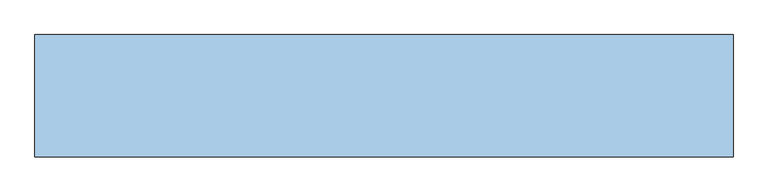
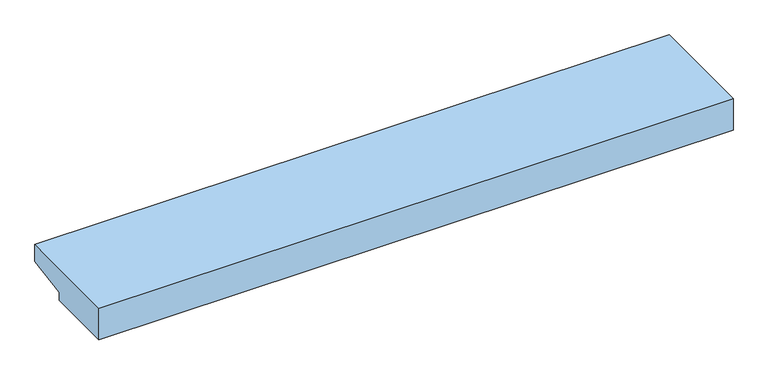
"""IFC4 building model written with IfcOpenShell, lengths in millimetres: window geometry, 린텔1 : 창대석."""

from ifc_helpers import new_model, si_unit, frame, origin, place, context, project, spatial, polyline, outline, extrude, source, transform, mapped, element, save


def window_50d48024(model_context):
    return source(origin(), model_context, "Body", "SweptSolid", [
        extrude(outline(polyline([(-195.0, 990.0), (435.0, 990.0), (435.0, 890.0), (195.0, 847.6815246), (195.0, 800.0), (-195.0, 800.0), (-195.0, 990.0)])), frame((-1800.0, 0.0, 0.0), z_axis=(1.0, 0.0, 0.0), x_axis=(0.0, 1.0, 0.0)), (0.0, 0.0, 1.0), 3600.0),
    ])


if __name__ == "__main__":
    model = new_model("IFC4")
    model_context = context("Model", 3, world=origin())
    ifc_project = project(units=[si_unit("LENGTHUNIT", "METRE", prefix="MILLI")], contexts=[model_context])
    site = spatial("IfcSite", under=ifc_project)
    building = spatial("IfcBuilding", under=site)
    placement = place(None, origin())
    window_shape = window_50d48024(model_context)
    element("IfcWindow", 1, ObjectType="린텔1 : 창대석", at=placement, inside=building, context=model_context, shape_type="MappedRepresentation", body=[
        mapped(window_shape, transform((0.0, 0.0, 0.0), x_axis=(1.0, 0.0, 0.0), y_axis=(0.0, 1.0, 0.0), z_axis=(0.0, 0.0, 1.0))),
    ])
    save(model, "model.ifc")

# Revit data of these elements
# Type "린텔1 : 창대석"
#   Type Mark = "200"
#   Analytic Construction = "<없음>"
#   두께 = 190 mm
#   돌출부두께 = 190 mm
#   돌출길이 = 240 mm
#   Height = 190 mm
#   Default Sill Height = 800 mm
#   Width = 3600 mm
#   Define Thermal Properties by = 1
#   Wall Closure = (empty or 0)
